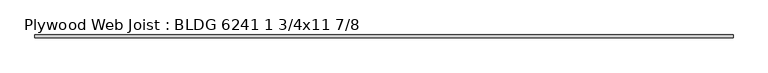
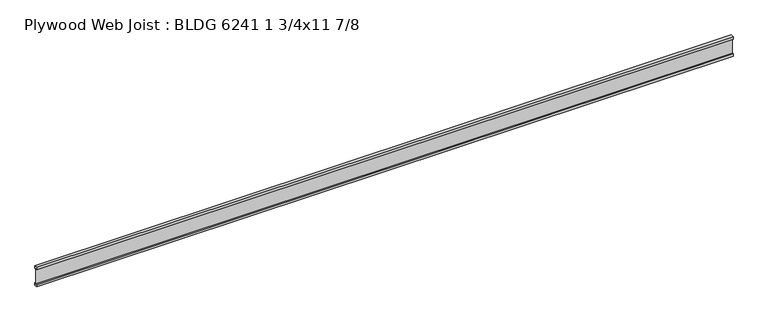
"""IFC4 building model written with IfcOpenShell, lengths in millimetres: beam geometry, Plywood Web Joist : BLDG 6241 1 3/4x11 7/8."""

from ifc_helpers import new_model, si_unit, frame, origin, place, context, project, spatial, polyline, outline, extrude, source, transform, mapped, element, save


def plywood_web_joist_bldg_6241_1_3_4x11_7_8_b749f0c8(model_context):
    return source(origin(), model_context, "Body", "SweptSolid", [
        extrude(outline(polyline([(-22.225, 150.8125), (22.225, 150.8125), (22.225, 112.7125), (4.7625, 112.7125), (4.7625, 119.0625), (-4.7625, 119.0625), (-4.7625, 112.7125), (-22.225, 112.7125), (-22.225, 150.8125)])), frame((-5041.9, 0.0, 0.0), z_axis=(1.0, 0.0, 0.0), x_axis=(0.0, 1.0, 0.0)), (0.0, 0.0, 1.0), 10083.8),
        extrude(outline(polyline([(22.225, -112.7125), (22.225, -150.8125), (-22.225, -150.8125), (-22.225, -112.7125), (-4.7625, -112.7125), (-4.7625, -118.3285374), (4.7625, -118.3285374), (4.7625, -112.7125), (22.225, -112.7125)])), frame((-5041.9, 0.0, 0.0), z_axis=(1.0, 0.0, 0.0), x_axis=(0.0, 1.0, 0.0)), (0.0, 0.0, 1.0), 10083.8),
        extrude(outline(polyline([(5041.9, 4.7625), (5041.9, -4.7625), (-5041.9, -4.7625), (-5041.9, 4.7625), (5041.9, 4.7625)])), frame((0.0, 0.0, -118.3285374), z_axis=(0.0, 0.0, 1.0), x_axis=(1.0, 0.0, 0.0)), (0.0, 0.0, 1.0), 237.3910374),
    ])


if __name__ == "__main__":
    model = new_model("IFC4")
    model_context = context("Model", 3, world=origin())
    ifc_project = project(units=[si_unit("LENGTHUNIT", "METRE", prefix="MILLI")], contexts=[model_context])
    site = spatial("IfcSite", under=ifc_project)
    building = spatial("IfcBuilding", under=site)
    placement = place(None, origin())
    plywood_web_joist_bldg_6241_1_3_4x11_7_8_shape = plywood_web_joist_bldg_6241_1_3_4x11_7_8_b749f0c8(model_context)
    element("IfcBeam", 1, ObjectType="Plywood Web Joist : BLDG 6241 1 3/4x11 7/8", at=placement, inside=building, context=model_context, shape_type="MappedRepresentation", body=[
        mapped(plywood_web_joist_bldg_6241_1_3_4x11_7_8_shape, transform((0.0, 0.0, 0.0), x_axis=(1.0, 0.0, 0.0), y_axis=(0.0, 1.0, 0.0), z_axis=(0.0, 0.0, 1.0))),
    ])
    save(model, "model.ifc")

# Revit data of these elements
# Type "Plywood Web Joist : BLDG 6241 1 3/4x11 7/8"
#   Assembly Code = "B10"
#   Length [instance default] = 5' - 0"
#   b = 0' - 1 3/4"
#   d = 0' - 11 7/8"
#   Structural Material [instance default] = Softwood, Lumber
# Element 1 (IfcBeam, "Plywood Web Joist : BLDG 6241 1 3/4x11 7/8")
#   Materials on its faces: "Softwood, Lumber"
# Materials
#   "Softwood, Lumber": class "Wood", colour RGB 223 192 134, transparency 0, Description = "Pinus Echinata", Cost = 0
